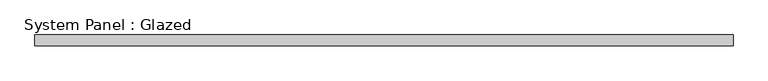
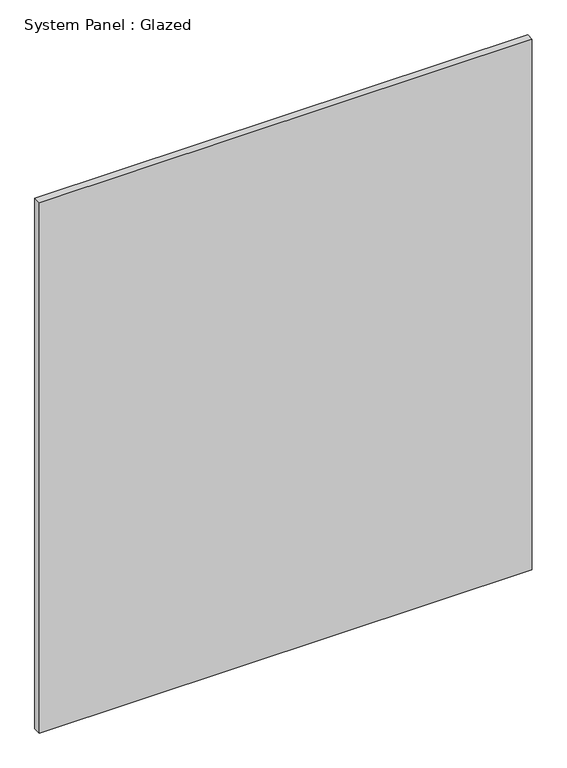
"""IFC4 building model written with IfcOpenShell, lengths in millimetres: plate geometry, System Panel : Glazed."""

from ifc_helpers import new_model, si_unit, origin, origin_with_axes, place, context, project, spatial, polyline, outline, extrude, source, transform, mapped, element, save


def system_panel_glazed_92ccea1f(model_context):
    return source(origin(), model_context, "Body", "SweptSolid", [
        extrude(outline(polyline([(807.8178526, 24.5), (-807.8178526, 24.5), (-807.8178526, 49.5), (807.8178526, 49.5), (807.8178526, 24.5)])), origin_with_axes(), (0.0, 0.0, 1.0), 1837.3779433),
    ])


if __name__ == "__main__":
    model = new_model("IFC4")
    model_context = context("Model", 3, world=origin())
    ifc_project = project(units=[si_unit("LENGTHUNIT", "METRE", prefix="MILLI")], contexts=[model_context])
    site = spatial("IfcSite", under=ifc_project)
    building = spatial("IfcBuilding", under=site)
    placement = place(None, origin())
    system_panel_glazed_shape = system_panel_glazed_92ccea1f(model_context)
    element("IfcPlate", 1, ObjectType="System Panel : Glazed", at=placement, inside=building, context=model_context, shape_type="MappedRepresentation", body=[
        mapped(system_panel_glazed_shape, transform((0.0, 0.0, 0.0), x_axis=(1.0, 0.0, 0.0), y_axis=(0.0, 1.0, 0.0), z_axis=(0.0, 0.0, 1.0))),
    ])
    save(model, "model.ifc")

# Revit data of these elements
# Element 1 (IfcPlate, "System Panel : Glazed")
#   Materials on its faces: "Glass"
# Materials
#   "Glass": class "Glass", colour RGB 218 227 224, transparency 0.85, Description = "Soda Lime Glass", Cost = 0
